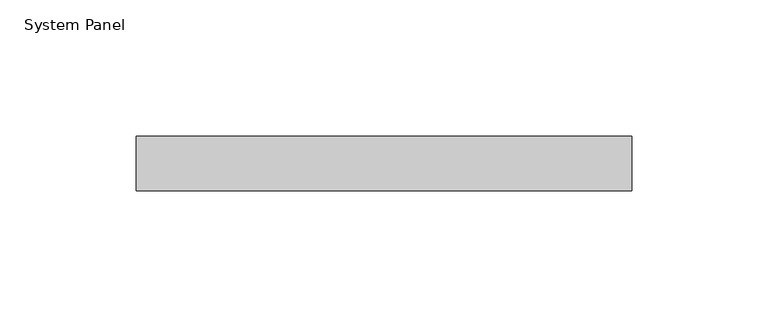
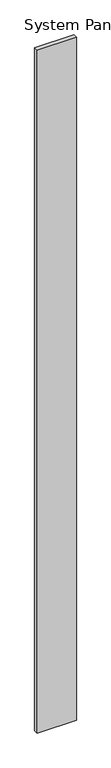
"""IFC4 building model written with IfcOpenShell, lengths in millimetres: plate geometry, System Panel : WWm-Glass-20mm-10mmOffset."""

from ifc_helpers import new_model, si_unit, origin, origin_with_axes, place, context, project, spatial, polyline, outline, extrude, source, transform, mapped, element, save


def system_panel_4ad90418(model_context):
    return source(origin(), model_context, "Body", "SweptSolid", [
        extrude(outline(polyline([(90.885636, 0.0), (-90.885636, 0.0), (-90.885636, 20.0), (90.885636, 20.0), (90.885636, 0.0)])), origin_with_axes(), (0.0, 0.0, 1.0), 3350.0),
    ])


if __name__ == "__main__":
    model = new_model("IFC4")
    model_context = context("Model", 3, world=origin())
    ifc_project = project(units=[si_unit("LENGTHUNIT", "METRE", prefix="MILLI")], contexts=[model_context])
    site = spatial("IfcSite", under=ifc_project)
    building = spatial("IfcBuilding", under=site)
    placement = place(None, origin())
    system_panel_shape = system_panel_4ad90418(model_context)
    element("IfcPlate", 1, ObjectType="System Panel : WWm-Glass-20mm-10mmOffset", at=placement, inside=building, context=model_context, shape_type="MappedRepresentation", body=[
        mapped(system_panel_shape, transform((0.0, 0.0, 0.0), x_axis=(1.0, 0.0, 0.0), y_axis=(0.0, 1.0, 0.0), z_axis=(0.0, 0.0, 1.0))),
    ])
    save(model, "model.ifc")

# Revit data of these elements
# Type "System Panel : WWm-Glass-20mm-10mmOffset"
#   Finish = ""
# Element 1 (IfcPlate, "System Panel : WWm-Glass-20mm-10mmOffset")
#   Materials on its faces: "WW-EC-GL-Storefront"
# Materials
#   "WW-EC-GL-Storefront": class "Glass", colour RGB 236 240 239, transparency 0.85, Description = "Storefront Glass", Cost = 0
